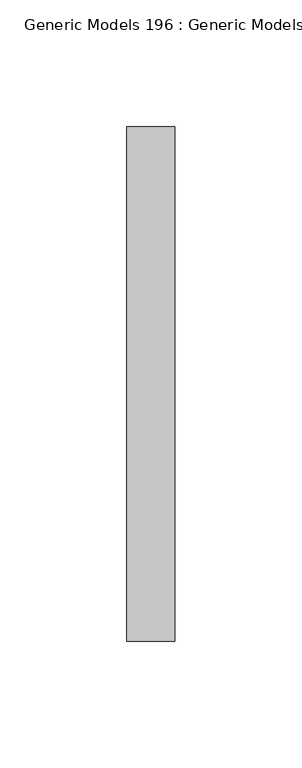
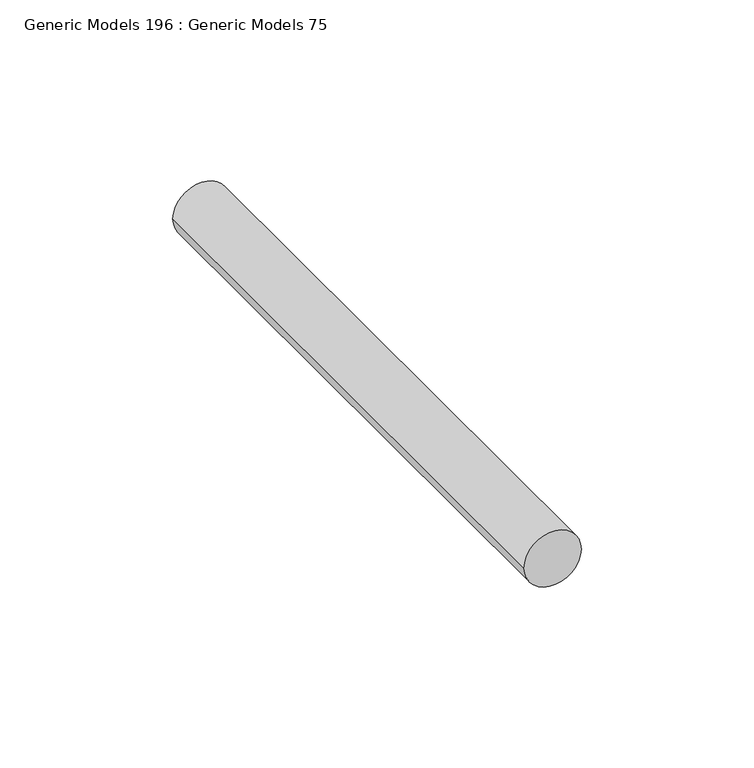
"""IFC4 building model written with IfcOpenShell, lengths in millimetres: proxy geometry, Generic Models 196 : Generic Models 75."""

from ifc_helpers import new_model, si_unit, point, frame, frame_2d, origin, place, context, project, spatial, circle_curve, trimmed, segment, composite_curve, outline, extrude, source, transform, mapped, element, save


def generic_models_196_generic_models_75_eeaa47ce(model_context):
    return source(origin(), model_context, "Body", "SweptSolid", [
        extrude(outline(composite_curve([segment(trimmed(circle_curve(frame_2d((271843.5, 31975.4096032)), 9.525), [point((271843.5, 31965.8846032))], [point((271843.5, 31984.9346032))], False, "CARTESIAN"), True, "CONTINUOUS"), segment(trimmed(circle_curve(frame_2d((271843.5, 31975.4096032)), 9.525), [point((271843.5, 31984.9346032))], [point((271843.5, 31965.8846032))], False, "CARTESIAN"), True, "CONTINUOUS")], self_intersect=False)), frame((0.0, 35188.2207942, 0.0), z_axis=(0.0, 1.0, 0.0), x_axis=(0.0, 0.0, 1.0)), (0.0, 0.0, 1.0), 203.2),
    ])


if __name__ == "__main__":
    model = new_model("IFC4")
    model_context = context("Model", 3, world=origin())
    ifc_project = project(units=[si_unit("LENGTHUNIT", "METRE", prefix="MILLI")], contexts=[model_context])
    site = spatial("IfcSite", under=ifc_project)
    building = spatial("IfcBuilding", under=site)
    placement = place(None, origin())
    generic_models_196_generic_models_75_shape = generic_models_196_generic_models_75_eeaa47ce(model_context)
    element("IfcBuildingElementProxy", 1, Name="Generic Models 196 : Generic Models 75", ObjectType="Generic Models 196 : Generic Models 75", at=placement, inside=building, context=model_context, shape_type="MappedRepresentation", body=[
        mapped(generic_models_196_generic_models_75_shape, transform((0.0, 0.0, 0.0), x_axis=(1.0, 0.0, 0.0), y_axis=(0.0, 1.0, 0.0), z_axis=(0.0, 0.0, 1.0))),
    ])
    save(model, "model.ifc")
